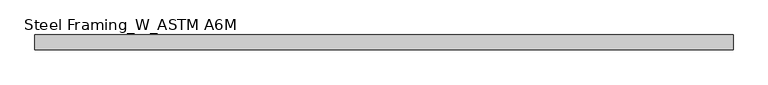
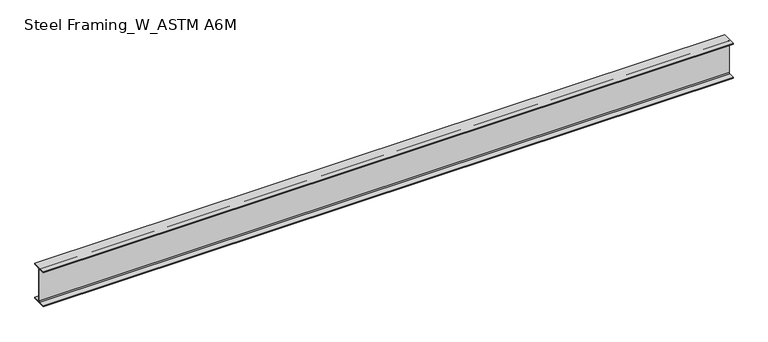
"""IFC4 building model written with IfcOpenShell, lengths in millimetres: beam geometry, Steel Framing_W_ASTM A6M : H_SB_AR_S02_W530x101_RB1."""

from ifc_helpers import new_model, si_unit, point, frame, frame_2d, origin, place, context, project, spatial, polyline, circle_curve, trimmed, segment, composite_curve, outline, extrude, source, transform, mapped, element, save


def steel_framing_w_astm_a6m_daca2dd2(model_context):
    return source(origin(), model_context, "Body", "SweptSolid", [
        extrude(outline(composite_curve([segment(polyline([(105.0, -250.6), (105.0, -268.0), (-105.0, -268.0), (-105.0, -250.6), (-18.25, -250.6)]), True, "CONTINUOUS"), segment(trimmed(circle_curve(frame_2d((-18.25, -237.8)), 12.8), [point((-18.25, -250.6))], [point((-5.45, -237.8))], True, "CARTESIAN"), True, "CONTINUOUS"), segment(polyline([(-5.45, -237.8), (-5.45, 237.8)]), True, "CONTINUOUS"), segment(trimmed(circle_curve(frame_2d((-18.25, 237.8)), 12.8), [point((-5.45, 237.8))], [point((-18.25, 250.6))], True, "CARTESIAN"), True, "CONTINUOUS"), segment(polyline([(-18.25, 250.6), (-105.0, 250.6), (-105.0, 268.0), (105.0, 268.0), (105.0, 250.6), (18.25, 250.6)]), True, "CONTINUOUS"), segment(trimmed(circle_curve(frame_2d((18.25, 237.8)), 12.8), [point((18.25, 250.6))], [point((5.45, 237.8))], True, "CARTESIAN"), True, "CONTINUOUS"), segment(polyline([(5.45, 237.8), (5.45, -237.8)]), True, "CONTINUOUS"), segment(trimmed(circle_curve(frame_2d((18.25, -237.8)), 12.8), [point((5.45, -237.8))], [point((18.25, -250.6))], True, "CARTESIAN"), True, "CONTINUOUS"), segment(polyline([(18.25, -250.6), (105.0, -250.6)]), True, "CONTINUOUS")], self_intersect=False)), frame((-4987.2, 0.0, 0.0), z_axis=(1.0, 0.0, 0.0), x_axis=(0.0, 1.0, 0.0)), (0.0, 0.0, 1.0), 9974.4),
    ])


if __name__ == "__main__":
    model = new_model("IFC4")
    model_context = context("Model", 3, world=origin())
    ifc_project = project(units=[si_unit("LENGTHUNIT", "METRE", prefix="MILLI")], contexts=[model_context])
    site = spatial("IfcSite", under=ifc_project)
    building = spatial("IfcBuilding", under=site)
    placement = place(None, origin())
    steel_framing_w_astm_a6m_shape = steel_framing_w_astm_a6m_daca2dd2(model_context)
    element("IfcBeam", 1, ObjectType="Steel Framing_W_ASTM A6M : H_SB_AR_S02_W530x101_RB1", at=placement, inside=building, context=model_context, shape_type="MappedRepresentation", body=[
        mapped(steel_framing_w_astm_a6m_shape, transform((0.0, 0.0, 0.0), x_axis=(1.0, 0.0, 0.0), y_axis=(0.0, 1.0, 0.0), z_axis=(0.0, 0.0, 1.0))),
    ])
    save(model, "model.ifc")

# Revit data of these elements
# Type "Steel Framing_W_ASTM A6M : H_SB_AR_S02_W530x101_RB1"
#   Type Mark = "RB1"
#   Section Name Key = "W21x68"
#   Width = 21.0 cm
#   Web Thickness = 1.09 cm
#   Web Fillet = 1.28 cm
#   Warping Constant = 1820000.0 cm⁶
#   Torsional Moment of Inertia = 102.00 cm⁴
#   Section Area = 129.0 cm²
#   Plastic Modulus weak axis = 400.0 cm³
#   Plastic Modulus strong axis = 2620.0 cm³
#   Perimeter = 1.87 m²/m
#   Nominal Weight = 101.00 kgf/m
#   Moment of Inertia weak axis = 2690.00 cm⁴
#   Moment of Inertia strong axis = 61600.00 cm⁴
#   Height = 53.6 cm
#   Flange Thickness = 1.74 cm
#   Elastic Modulus weak axis = 257.0 cm³
#   Elastic Modulus strong axis = 2290.0 cm³
#   Centroid Vertical = 26.8 cm
#   Centroid Horizontal = 10.5 cm
#   Length [instance default] = 1500 mm
#   Structural Material [instance default] = Steel, 45-345
#   Bolt Spacing = 0
#   Assembly Code = ""
# Element 1 (IfcBeam, "Steel Framing_W_ASTM A6M : H_SB_AR_S02_W530x101_RB1")
#   Materials on its faces: "Steel, 45-345"
# Materials
#   "Steel, 45-345": class "Metal", colour RGB 189 187 185, transparency 0, Description = "Steel 345 MPa", Cost = 0
